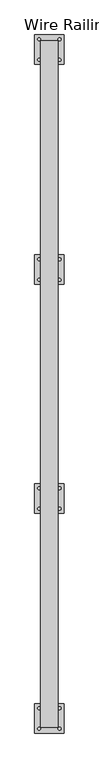
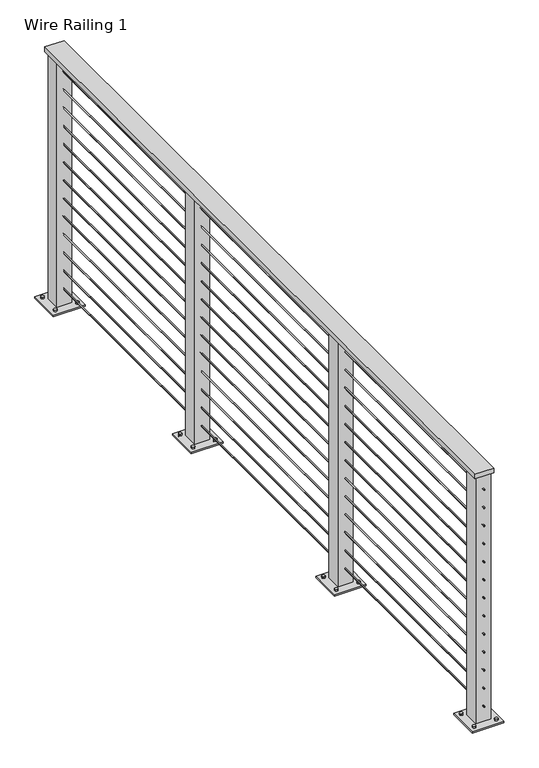
"""IFC4 building model written with IfcOpenShell, lengths in millimetres: railing geometry, Wire Railing 1."""

from ifc_helpers import new_model, si_unit, point, frame, frame_2d, origin, place, context, project, spatial, polyline, circle_curve, trimmed, segment, composite_curve, outline, extrude, source, transform, mapped, element, save


def wire_railing_1_db42b38e(model_context):
    return source(origin(), model_context, "Body", "SweptSolid", [
        extrude(outline(polyline([(-9075.1938771, -3058.3548735), (-9151.3938771, -3058.3548735), (-9151.3938771, -84.9595308), (-9075.1938771, -84.9595308), (-9075.1938771, -3058.3548735)])), frame((0.0, 0.0, 4502.15), z_axis=(0.0, 0.0, 1.0), x_axis=(1.0, 0.0, 0.0)), (0.0, 0.0, 1.0), 19.05),
        extrude(outline(composite_curve([segment(trimmed(circle_curve(frame_2d((4442.61875, -9113.2938771)), 2.38125), [point((4442.61875, -9115.6751271))], [point((4442.61875, -9110.9126271))], False, "CARTESIAN"), True, "CONTINUOUS"), segment(trimmed(circle_curve(frame_2d((4442.61875, -9113.2938771)), 2.38125), [point((4442.61875, -9110.9126271))], [point((4442.61875, -9115.6751271))], False, "CARTESIAN"), True, "CONTINUOUS")], self_intersect=False)), frame((0.0, -3058.3548735, 0.0), z_axis=(0.0, 1.0, 0.0), x_axis=(0.0, 0.0, 1.0)), (0.0, 0.0, 1.0), 2973.3953427),
        extrude(outline(composite_curve([segment(trimmed(circle_curve(frame_2d((4366.41875, -9113.2938771)), 2.38125), [point((4366.41875, -9115.6751271))], [point((4366.41875, -9110.9126271))], False, "CARTESIAN"), True, "CONTINUOUS"), segment(trimmed(circle_curve(frame_2d((4366.41875, -9113.2938771)), 2.38125), [point((4366.41875, -9110.9126271))], [point((4366.41875, -9115.6751271))], False, "CARTESIAN"), True, "CONTINUOUS")], self_intersect=False)), frame((0.0, -3058.3548735, 0.0), z_axis=(0.0, 1.0, 0.0), x_axis=(0.0, 0.0, 1.0)), (0.0, 0.0, 1.0), 2973.3953427),
        extrude(outline(composite_curve([segment(trimmed(circle_curve(frame_2d((4290.21875, -9113.2938771)), 2.38125), [point((4290.21875, -9115.6751271))], [point((4290.21875, -9110.9126271))], False, "CARTESIAN"), True, "CONTINUOUS"), segment(trimmed(circle_curve(frame_2d((4290.21875, -9113.2938771)), 2.38125), [point((4290.21875, -9110.9126271))], [point((4290.21875, -9115.6751271))], False, "CARTESIAN"), True, "CONTINUOUS")], self_intersect=False)), frame((0.0, -3058.3548735, 0.0), z_axis=(0.0, 1.0, 0.0), x_axis=(0.0, 0.0, 1.0)), (0.0, 0.0, 1.0), 2973.3953427),
        extrude(outline(composite_curve([segment(trimmed(circle_curve(frame_2d((4214.01875, -9113.2938771)), 2.38125), [point((4214.01875, -9115.6751271))], [point((4214.01875, -9110.9126271))], False, "CARTESIAN"), True, "CONTINUOUS"), segment(trimmed(circle_curve(frame_2d((4214.01875, -9113.2938771)), 2.38125), [point((4214.01875, -9110.9126271))], [point((4214.01875, -9115.6751271))], False, "CARTESIAN"), True, "CONTINUOUS")], self_intersect=False)), frame((0.0, -3058.3548735, 0.0), z_axis=(0.0, 1.0, 0.0), x_axis=(0.0, 0.0, 1.0)), (0.0, 0.0, 1.0), 2973.3953427),
        extrude(outline(composite_curve([segment(trimmed(circle_curve(frame_2d((4137.81875, -9113.2938771)), 2.38125), [point((4137.81875, -9115.6751271))], [point((4137.81875, -9110.9126271))], False, "CARTESIAN"), True, "CONTINUOUS"), segment(trimmed(circle_curve(frame_2d((4137.81875, -9113.2938771)), 2.38125), [point((4137.81875, -9110.9126271))], [point((4137.81875, -9115.6751271))], False, "CARTESIAN"), True, "CONTINUOUS")], self_intersect=False)), frame((0.0, -3058.3548735, 0.0), z_axis=(0.0, 1.0, 0.0), x_axis=(0.0, 0.0, 1.0)), (0.0, 0.0, 1.0), 2973.3953427),
        extrude(outline(composite_curve([segment(trimmed(circle_curve(frame_2d((4061.61875, -9113.2938771)), 2.38125), [point((4061.61875, -9115.6751271))], [point((4061.61875, -9110.9126271))], False, "CARTESIAN"), True, "CONTINUOUS"), segment(trimmed(circle_curve(frame_2d((4061.61875, -9113.2938771)), 2.38125), [point((4061.61875, -9110.9126271))], [point((4061.61875, -9115.6751271))], False, "CARTESIAN"), True, "CONTINUOUS")], self_intersect=False)), frame((0.0, -3058.3548735, 0.0), z_axis=(0.0, 1.0, 0.0), x_axis=(0.0, 0.0, 1.0)), (0.0, 0.0, 1.0), 2973.3953427),
        extrude(outline(composite_curve([segment(trimmed(circle_curve(frame_2d((3985.41875, -9113.2938771)), 2.38125), [point((3985.41875, -9115.6751271))], [point((3985.41875, -9110.9126271))], False, "CARTESIAN"), True, "CONTINUOUS"), segment(trimmed(circle_curve(frame_2d((3985.41875, -9113.2938771)), 2.38125), [point((3985.41875, -9110.9126271))], [point((3985.41875, -9115.6751271))], False, "CARTESIAN"), True, "CONTINUOUS")], self_intersect=False)), frame((0.0, -3058.3548735, 0.0), z_axis=(0.0, 1.0, 0.0), x_axis=(0.0, 0.0, 1.0)), (0.0, 0.0, 1.0), 2973.3953427),
        extrude(outline(composite_curve([segment(trimmed(circle_curve(frame_2d((3909.21875, -9113.2938771)), 2.38125), [point((3909.21875, -9115.6751271))], [point((3909.21875, -9110.9126271))], False, "CARTESIAN"), True, "CONTINUOUS"), segment(trimmed(circle_curve(frame_2d((3909.21875, -9113.2938771)), 2.38125), [point((3909.21875, -9110.9126271))], [point((3909.21875, -9115.6751271))], False, "CARTESIAN"), True, "CONTINUOUS")], self_intersect=False)), frame((0.0, -3058.3548735, 0.0), z_axis=(0.0, 1.0, 0.0), x_axis=(0.0, 0.0, 1.0)), (0.0, 0.0, 1.0), 2973.3953427),
        extrude(outline(composite_curve([segment(trimmed(circle_curve(frame_2d((3833.01875, -9113.2938771)), 2.38125), [point((3833.01875, -9115.6751271))], [point((3833.01875, -9110.9126271))], False, "CARTESIAN"), True, "CONTINUOUS"), segment(trimmed(circle_curve(frame_2d((3833.01875, -9113.2938771)), 2.38125), [point((3833.01875, -9110.9126271))], [point((3833.01875, -9115.6751271))], False, "CARTESIAN"), True, "CONTINUOUS")], self_intersect=False)), frame((0.0, -3058.3548735, 0.0), z_axis=(0.0, 1.0, 0.0), x_axis=(0.0, 0.0, 1.0)), (0.0, 0.0, 1.0), 2973.3953427),
        extrude(outline(composite_curve([segment(trimmed(circle_curve(frame_2d((3756.81875, -9113.2938771)), 2.38125), [point((3756.81875, -9115.6751271))], [point((3756.81875, -9110.9126271))], False, "CARTESIAN"), True, "CONTINUOUS"), segment(trimmed(circle_curve(frame_2d((3756.81875, -9113.2938771)), 2.38125), [point((3756.81875, -9110.9126271))], [point((3756.81875, -9115.6751271))], False, "CARTESIAN"), True, "CONTINUOUS")], self_intersect=False)), frame((0.0, -3058.3548735, 0.0), z_axis=(0.0, 1.0, 0.0), x_axis=(0.0, 0.0, 1.0)), (0.0, 0.0, 1.0), 2973.3953427),
        extrude(outline(composite_curve([segment(trimmed(circle_curve(frame_2d((3680.61875, -9113.2938771)), 2.38125), [point((3680.61875, -9115.6751271))], [point((3680.61875, -9110.9126271))], False, "CARTESIAN"), True, "CONTINUOUS"), segment(trimmed(circle_curve(frame_2d((3680.61875, -9113.2938771)), 2.38125), [point((3680.61875, -9110.9126271))], [point((3680.61875, -9115.6751271))], False, "CARTESIAN"), True, "CONTINUOUS")], self_intersect=False)), frame((0.0, -3058.3548735, 0.0), z_axis=(0.0, 1.0, 0.0), x_axis=(0.0, 0.0, 1.0)), (0.0, 0.0, 1.0), 2973.3953427),
        extrude(outline(composite_curve([segment(trimmed(circle_curve(frame_2d((3604.41875, -9113.2938771)), 2.38125), [point((3604.41875, -9115.6751271))], [point((3604.41875, -9110.9126271))], False, "CARTESIAN"), True, "CONTINUOUS"), segment(trimmed(circle_curve(frame_2d((3604.41875, -9113.2938771)), 2.38125), [point((3604.41875, -9110.9126271))], [point((3604.41875, -9115.6751271))], False, "CARTESIAN"), True, "CONTINUOUS")], self_intersect=False)), frame((0.0, -3058.3548735, 0.0), z_axis=(0.0, 1.0, 0.0), x_axis=(0.0, 0.0, 1.0)), (0.0, 0.0, 1.0), 2973.3953427),
        extrude(outline(composite_curve([segment(trimmed(circle_curve(frame_2d((3528.21875, -9113.2938771)), 2.38125), [point((3528.21875, -9115.6751271))], [point((3528.21875, -9110.9126271))], False, "CARTESIAN"), True, "CONTINUOUS"), segment(trimmed(circle_curve(frame_2d((3528.21875, -9113.2938771)), 2.38125), [point((3528.21875, -9110.9126271))], [point((3528.21875, -9115.6751271))], False, "CARTESIAN"), True, "CONTINUOUS")], self_intersect=False)), frame((0.0, -3058.3548735, 0.0), z_axis=(0.0, 1.0, 0.0), x_axis=(0.0, 0.0, 1.0)), (0.0, 0.0, 1.0), 2973.3953427),
        extrude(outline(composite_curve([segment(trimmed(circle_curve(frame_2d((-9068.8438771, -1120.5413117)), 6.35), [point((-9062.4938771, -1120.5413117))], [point((-9075.1938771, -1120.5413117))], False, "CARTESIAN"), True, "CONTINUOUS"), segment(trimmed(circle_curve(frame_2d((-9068.8438771, -1120.5413117)), 6.35), [point((-9075.1938771, -1120.5413117))], [point((-9062.4938771, -1120.5413117))], False, "CARTESIAN"), True, "CONTINUOUS")], self_intersect=False)), frame((0.0, 0.0, 3454.4), z_axis=(0.0, 0.0, 1.0), x_axis=(1.0, 0.0, 0.0)), (0.0, 0.0, 1.0), 12.7),
        extrude(outline(composite_curve([segment(trimmed(circle_curve(frame_2d((-9157.7438771, -1120.5413117)), 6.35), [point((-9151.3938771, -1120.5413117))], [point((-9164.0938771, -1120.5413117))], False, "CARTESIAN"), True, "CONTINUOUS"), segment(trimmed(circle_curve(frame_2d((-9157.7438771, -1120.5413117)), 6.35), [point((-9164.0938771, -1120.5413117))], [point((-9151.3938771, -1120.5413117))], False, "CARTESIAN"), True, "CONTINUOUS")], self_intersect=False)), frame((0.0, 0.0, 3454.4), z_axis=(0.0, 0.0, 1.0), x_axis=(1.0, 0.0, 0.0)), (0.0, 0.0, 1.0), 12.7),
        extrude(outline(composite_curve([segment(trimmed(circle_curve(frame_2d((-9068.8438771, -1031.6413117)), 6.35), [point((-9062.4938771, -1031.6413117))], [point((-9075.1938771, -1031.6413117))], False, "CARTESIAN"), True, "CONTINUOUS"), segment(trimmed(circle_curve(frame_2d((-9068.8438771, -1031.6413117)), 6.35), [point((-9075.1938771, -1031.6413117))], [point((-9062.4938771, -1031.6413117))], False, "CARTESIAN"), True, "CONTINUOUS")], self_intersect=False)), frame((0.0, 0.0, 3454.4), z_axis=(0.0, 0.0, 1.0), x_axis=(1.0, 0.0, 0.0)), (0.0, 0.0, 1.0), 12.7),
        extrude(outline(composite_curve([segment(trimmed(circle_curve(frame_2d((-9157.7438771, -1031.6413117)), 6.35), [point((-9151.3938771, -1031.6413117))], [point((-9164.0938771, -1031.6413117))], False, "CARTESIAN"), True, "CONTINUOUS"), segment(trimmed(circle_curve(frame_2d((-9157.7438771, -1031.6413117)), 6.35), [point((-9164.0938771, -1031.6413117))], [point((-9151.3938771, -1031.6413117))], False, "CARTESIAN"), True, "CONTINUOUS")], self_intersect=False)), frame((0.0, 0.0, 3454.4), z_axis=(0.0, 0.0, 1.0), x_axis=(1.0, 0.0, 0.0)), (0.0, 0.0, 1.0), 12.7),
        extrude(outline(polyline([(-9176.7938771, -1139.5913117), (-9176.7938771, -1012.5913117), (-9049.7938771, -1012.5913117), (-9049.7938771, -1139.5913117), (-9176.7938771, -1139.5913117)])), frame((0.0, 0.0, 3454.4), z_axis=(0.0, 0.0, 1.0), x_axis=(1.0, 0.0, 0.0)), (0.0, 0.0, 1.0), 6.35),
        extrude(outline(polyline([(-9143.4563771, -1106.2538117), (-9143.4563771, -1045.9288117), (-9083.1313771, -1045.9288117), (-9083.1313771, -1106.2538117), (-9143.4563771, -1106.2538117)]), holes=[polyline([(-9137.1063771, -1099.9038117), (-9089.4813771, -1099.9038117), (-9089.4813771, -1052.2788117), (-9137.1063771, -1052.2788117), (-9137.1063771, -1099.9038117)])]), frame((0.0, 0.0, 3454.4), z_axis=(0.0, 0.0, 1.0), x_axis=(1.0, 0.0, 0.0)), (0.0, 0.0, 1.0), 1047.75),
        extrude(outline(composite_curve([segment(trimmed(circle_curve(frame_2d((-9068.8438771, -2111.6730926)), 6.35), [point((-9062.4938771, -2111.6730926))], [point((-9075.1938771, -2111.6730926))], False, "CARTESIAN"), True, "CONTINUOUS"), segment(trimmed(circle_curve(frame_2d((-9068.8438771, -2111.6730926)), 6.35), [point((-9075.1938771, -2111.6730926))], [point((-9062.4938771, -2111.6730926))], False, "CARTESIAN"), True, "CONTINUOUS")], self_intersect=False)), frame((0.0, 0.0, 3454.4), z_axis=(0.0, 0.0, 1.0), x_axis=(1.0, 0.0, 0.0)), (0.0, 0.0, 1.0), 12.7),
        extrude(outline(composite_curve([segment(trimmed(circle_curve(frame_2d((-9157.7438771, -2111.6730926)), 6.35), [point((-9151.3938771, -2111.6730926))], [point((-9164.0938771, -2111.6730926))], False, "CARTESIAN"), True, "CONTINUOUS"), segment(trimmed(circle_curve(frame_2d((-9157.7438771, -2111.6730926)), 6.35), [point((-9164.0938771, -2111.6730926))], [point((-9151.3938771, -2111.6730926))], False, "CARTESIAN"), True, "CONTINUOUS")], self_intersect=False)), frame((0.0, 0.0, 3454.4), z_axis=(0.0, 0.0, 1.0), x_axis=(1.0, 0.0, 0.0)), (0.0, 0.0, 1.0), 12.7),
        extrude(outline(composite_curve([segment(trimmed(circle_curve(frame_2d((-9068.8438771, -2022.7730926)), 6.35), [point((-9062.4938771, -2022.7730926))], [point((-9075.1938771, -2022.7730926))], False, "CARTESIAN"), True, "CONTINUOUS"), segment(trimmed(circle_curve(frame_2d((-9068.8438771, -2022.7730926)), 6.35), [point((-9075.1938771, -2022.7730926))], [point((-9062.4938771, -2022.7730926))], False, "CARTESIAN"), True, "CONTINUOUS")], self_intersect=False)), frame((0.0, 0.0, 3454.4), z_axis=(0.0, 0.0, 1.0), x_axis=(1.0, 0.0, 0.0)), (0.0, 0.0, 1.0), 12.7),
        extrude(outline(composite_curve([segment(trimmed(circle_curve(frame_2d((-9157.7438771, -2022.7730926)), 6.35), [point((-9151.3938771, -2022.7730926))], [point((-9164.0938771, -2022.7730926))], False, "CARTESIAN"), True, "CONTINUOUS"), segment(trimmed(circle_curve(frame_2d((-9157.7438771, -2022.7730926)), 6.35), [point((-9164.0938771, -2022.7730926))], [point((-9151.3938771, -2022.7730926))], False, "CARTESIAN"), True, "CONTINUOUS")], self_intersect=False)), frame((0.0, 0.0, 3454.4), z_axis=(0.0, 0.0, 1.0), x_axis=(1.0, 0.0, 0.0)), (0.0, 0.0, 1.0), 12.7),
        extrude(outline(polyline([(-9176.7938771, -2130.7230926), (-9176.7938771, -2003.7230926), (-9049.7938771, -2003.7230926), (-9049.7938771, -2130.7230926), (-9176.7938771, -2130.7230926)])), frame((0.0, 0.0, 3454.4), z_axis=(0.0, 0.0, 1.0), x_axis=(1.0, 0.0, 0.0)), (0.0, 0.0, 1.0), 6.35),
        extrude(outline(polyline([(-9143.4563771, -2097.3855926), (-9143.4563771, -2037.0605926), (-9083.1313771, -2037.0605926), (-9083.1313771, -2097.3855926), (-9143.4563771, -2097.3855926)]), holes=[polyline([(-9137.1063771, -2091.0355926), (-9089.4813771, -2091.0355926), (-9089.4813771, -2043.4105926), (-9137.1063771, -2043.4105926), (-9137.1063771, -2091.0355926)])]), frame((0.0, 0.0, 3454.4), z_axis=(0.0, 0.0, 1.0), x_axis=(1.0, 0.0, 0.0)), (0.0, 0.0, 1.0), 1047.75),
        extrude(outline(composite_curve([segment(trimmed(circle_curve(frame_2d((-9068.8438771, -167.5095308)), 6.35), [point((-9062.4938771, -167.5095308))], [point((-9075.1938771, -167.5095308))], False, "CARTESIAN"), True, "CONTINUOUS"), segment(trimmed(circle_curve(frame_2d((-9068.8438771, -167.5095308)), 6.35), [point((-9075.1938771, -167.5095308))], [point((-9062.4938771, -167.5095308))], False, "CARTESIAN"), True, "CONTINUOUS")], self_intersect=False)), frame((0.0, 0.0, 3454.4), z_axis=(0.0, 0.0, 1.0), x_axis=(1.0, 0.0, 0.0)), (0.0, 0.0, 1.0), 12.7),
        extrude(outline(composite_curve([segment(trimmed(circle_curve(frame_2d((-9157.7438771, -167.5095308)), 6.35), [point((-9151.3938771, -167.5095308))], [point((-9164.0938771, -167.5095308))], False, "CARTESIAN"), True, "CONTINUOUS"), segment(trimmed(circle_curve(frame_2d((-9157.7438771, -167.5095308)), 6.35), [point((-9164.0938771, -167.5095308))], [point((-9151.3938771, -167.5095308))], False, "CARTESIAN"), True, "CONTINUOUS")], self_intersect=False)), frame((0.0, 0.0, 3454.4), z_axis=(0.0, 0.0, 1.0), x_axis=(1.0, 0.0, 0.0)), (0.0, 0.0, 1.0), 12.7),
        extrude(outline(composite_curve([segment(trimmed(circle_curve(frame_2d((-9068.8438771, -78.6095308)), 6.35), [point((-9062.4938771, -78.6095308))], [point((-9075.1938771, -78.6095308))], False, "CARTESIAN"), True, "CONTINUOUS"), segment(trimmed(circle_curve(frame_2d((-9068.8438771, -78.6095308)), 6.35), [point((-9075.1938771, -78.6095308))], [point((-9062.4938771, -78.6095308))], False, "CARTESIAN"), True, "CONTINUOUS")], self_intersect=False)), frame((0.0, 0.0, 3454.4), z_axis=(0.0, 0.0, 1.0), x_axis=(1.0, 0.0, 0.0)), (0.0, 0.0, 1.0), 12.7),
        extrude(outline(composite_curve([segment(trimmed(circle_curve(frame_2d((-9157.7438771, -78.6095308)), 6.35), [point((-9151.3938771, -78.6095308))], [point((-9164.0938771, -78.6095308))], False, "CARTESIAN"), True, "CONTINUOUS"), segment(trimmed(circle_curve(frame_2d((-9157.7438771, -78.6095308)), 6.35), [point((-9164.0938771, -78.6095308))], [point((-9151.3938771, -78.6095308))], False, "CARTESIAN"), True, "CONTINUOUS")], self_intersect=False)), frame((0.0, 0.0, 3454.4), z_axis=(0.0, 0.0, 1.0), x_axis=(1.0, 0.0, 0.0)), (0.0, 0.0, 1.0), 12.7),
        extrude(outline(polyline([(-9176.7938771, -186.5595308), (-9176.7938771, -59.5595308), (-9049.7938771, -59.5595308), (-9049.7938771, -186.5595308), (-9176.7938771, -186.5595308)])), frame((0.0, 0.0, 3454.4), z_axis=(0.0, 0.0, 1.0), x_axis=(1.0, 0.0, 0.0)), (0.0, 0.0, 1.0), 6.35),
        extrude(outline(polyline([(-9143.4563771, -153.2220308), (-9143.4563771, -92.8970308), (-9083.1313771, -92.8970308), (-9083.1313771, -153.2220308), (-9143.4563771, -153.2220308)]), holes=[polyline([(-9137.1063771, -146.8720308), (-9089.4813771, -146.8720308), (-9089.4813771, -99.2470308), (-9137.1063771, -99.2470308), (-9137.1063771, -146.8720308)])]), frame((0.0, 0.0, 3454.4), z_axis=(0.0, 0.0, 1.0), x_axis=(1.0, 0.0, 0.0)), (0.0, 0.0, 1.0), 1047.75),
        extrude(outline(composite_curve([segment(trimmed(circle_curve(frame_2d((-9068.8438771, -3064.7048735)), 6.35), [point((-9062.4938771, -3064.7048735))], [point((-9075.1938771, -3064.7048735))], False, "CARTESIAN"), True, "CONTINUOUS"), segment(trimmed(circle_curve(frame_2d((-9068.8438771, -3064.7048735)), 6.35), [point((-9075.1938771, -3064.7048735))], [point((-9062.4938771, -3064.7048735))], False, "CARTESIAN"), True, "CONTINUOUS")], self_intersect=False)), frame((0.0, 0.0, 3454.4), z_axis=(0.0, 0.0, 1.0), x_axis=(1.0, 0.0, 0.0)), (0.0, 0.0, 1.0), 12.7),
        extrude(outline(composite_curve([segment(trimmed(circle_curve(frame_2d((-9157.7438771, -3064.7048735)), 6.35), [point((-9151.3938771, -3064.7048735))], [point((-9164.0938771, -3064.7048735))], False, "CARTESIAN"), True, "CONTINUOUS"), segment(trimmed(circle_curve(frame_2d((-9157.7438771, -3064.7048735)), 6.35), [point((-9164.0938771, -3064.7048735))], [point((-9151.3938771, -3064.7048735))], False, "CARTESIAN"), True, "CONTINUOUS")], self_intersect=False)), frame((0.0, 0.0, 3454.4), z_axis=(0.0, 0.0, 1.0), x_axis=(1.0, 0.0, 0.0)), (0.0, 0.0, 1.0), 12.7),
        extrude(outline(composite_curve([segment(trimmed(circle_curve(frame_2d((-9068.8438771, -2975.8048735)), 6.35), [point((-9062.4938771, -2975.8048735))], [point((-9075.1938771, -2975.8048735))], False, "CARTESIAN"), True, "CONTINUOUS"), segment(trimmed(circle_curve(frame_2d((-9068.8438771, -2975.8048735)), 6.35), [point((-9075.1938771, -2975.8048735))], [point((-9062.4938771, -2975.8048735))], False, "CARTESIAN"), True, "CONTINUOUS")], self_intersect=False)), frame((0.0, 0.0, 3454.4), z_axis=(0.0, 0.0, 1.0), x_axis=(1.0, 0.0, 0.0)), (0.0, 0.0, 1.0), 12.7),
        extrude(outline(composite_curve([segment(trimmed(circle_curve(frame_2d((-9157.7438771, -2975.8048735)), 6.35), [point((-9151.3938771, -2975.8048735))], [point((-9164.0938771, -2975.8048735))], False, "CARTESIAN"), True, "CONTINUOUS"), segment(trimmed(circle_curve(frame_2d((-9157.7438771, -2975.8048735)), 6.35), [point((-9164.0938771, -2975.8048735))], [point((-9151.3938771, -2975.8048735))], False, "CARTESIAN"), True, "CONTINUOUS")], self_intersect=False)), frame((0.0, 0.0, 3454.4), z_axis=(0.0, 0.0, 1.0), x_axis=(1.0, 0.0, 0.0)), (0.0, 0.0, 1.0), 12.7),
        extrude(outline(polyline([(-9176.7938771, -3083.7548735), (-9176.7938771, -2956.7548735), (-9049.7938771, -2956.7548735), (-9049.7938771, -3083.7548735), (-9176.7938771, -3083.7548735)])), frame((0.0, 0.0, 3454.4), z_axis=(0.0, 0.0, 1.0), x_axis=(1.0, 0.0, 0.0)), (0.0, 0.0, 1.0), 6.35),
        extrude(outline(polyline([(-9143.4563771, -3050.4173735), (-9143.4563771, -2990.0923735), (-9083.1313771, -2990.0923735), (-9083.1313771, -3050.4173735), (-9143.4563771, -3050.4173735)]), holes=[polyline([(-9137.1063771, -3044.0673735), (-9089.4813771, -3044.0673735), (-9089.4813771, -2996.4423735), (-9137.1063771, -2996.4423735), (-9137.1063771, -3044.0673735)])]), frame((0.0, 0.0, 3454.4), z_axis=(0.0, 0.0, 1.0), x_axis=(1.0, 0.0, 0.0)), (0.0, 0.0, 1.0), 1047.75),
    ])


if __name__ == "__main__":
    model = new_model("IFC4")
    model_context = context("Model", 3, world=origin())
    ifc_project = project(units=[si_unit("LENGTHUNIT", "METRE", prefix="MILLI")], contexts=[model_context])
    site = spatial("IfcSite", under=ifc_project)
    building = spatial("IfcBuilding", under=site)
    placement = place(None, origin())
    wire_railing_1_shape = wire_railing_1_db42b38e(model_context)
    element("IfcRailing", 1, ObjectType="Wire Railing 1", at=placement, inside=building, context=model_context, shape_type="MappedRepresentation", body=[
        mapped(wire_railing_1_shape, transform((0.0, 0.0, 0.0), x_axis=(1.0, 0.0, 0.0), y_axis=(0.0, 1.0, 0.0), z_axis=(0.0, 0.0, 1.0))),
    ])
    save(model, "model.ifc")

# Revit data of these elements
# Element 1 (IfcRailing, "Wire Railing 1")
#   Materials on its faces: "Metal - Kawneer - Aluminum"
# Materials
#   "Metal - Kawneer - Aluminum": class "Metal", colour RGB 244 244 244, transparency 0, Manufacturer = "Kawneer", URL = "http://www.kawneer.com/kawneer/north_america/en/home.asp", Cost = 0
